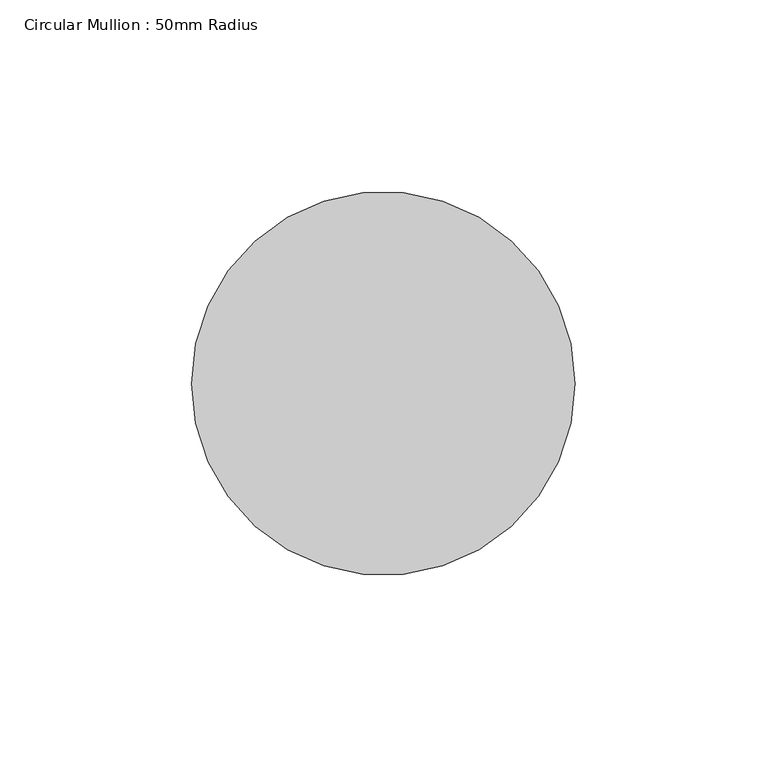
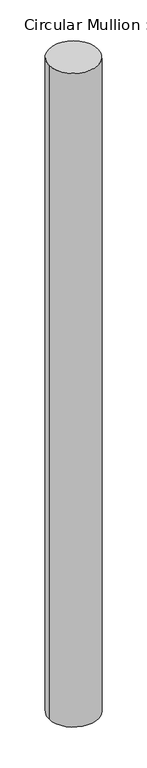
"""IFC4 building model written with IfcOpenShell, lengths in millimetres: member geometry, Circular Mullion : 50mm Radius."""

from ifc_helpers import new_model, si_unit, point, frame, origin, origin_2d, place, context, project, spatial, circle_curve, trimmed, segment, composite_curve, outline, extrude, source, transform, mapped, element, save


def circular_mullion_50mm_radius_d3639100(model_context):
    return source(origin(), model_context, "Body", "SweptSolid", [
        extrude(outline(composite_curve([segment(trimmed(circle_curve(origin_2d(), 50.0), [point((50.0, 0.0))], [point((-50.0, 0.0))], False, "CARTESIAN"), True, "CONTINUOUS"), segment(trimmed(circle_curve(origin_2d(), 50.0), [point((-50.0, 0.0))], [point((50.0, 0.0))], False, "CARTESIAN"), True, "CONTINUOUS")], self_intersect=False)), frame((0.0, 0.0, -1404.0355883), z_axis=(0.0, 0.0, 1.0), x_axis=(1.0, 0.0, 0.0)), (0.0, 0.0, 1.0), 1404.0355883),
    ])


if __name__ == "__main__":
    model = new_model("IFC4")
    model_context = context("Model", 3, world=origin())
    ifc_project = project(units=[si_unit("LENGTHUNIT", "METRE", prefix="MILLI")], contexts=[model_context])
    site = spatial("IfcSite", under=ifc_project)
    building = spatial("IfcBuilding", under=site)
    placement = place(None, origin())
    circular_mullion_50mm_radius_shape = circular_mullion_50mm_radius_d3639100(model_context)
    element("IfcMember", 1, ObjectType="Circular Mullion : 50mm Radius", at=placement, inside=building, context=model_context, shape_type="MappedRepresentation", body=[
        mapped(circular_mullion_50mm_radius_shape, transform((0.0, 0.0, 0.0), x_axis=(1.0, 0.0, 0.0), y_axis=(0.0, 1.0, 0.0), z_axis=(0.0, 0.0, 1.0))),
    ])
    save(model, "model.ifc")

# Revit data of these elements
# Type "Circular Mullion : 50mm Radius"
#   built-in parameter 1007350 = 0.164042 (stored number, unit not read)
# Element 1 (IfcMember, "Circular Mullion : 50mm Radius")
#   Materials on its faces: "Aluminium"
# Materials
#   "Aluminium": class "Metal", colour RGB 247 247 247, transparency 0, Description = "Aluminium 6061", Cost = 0
